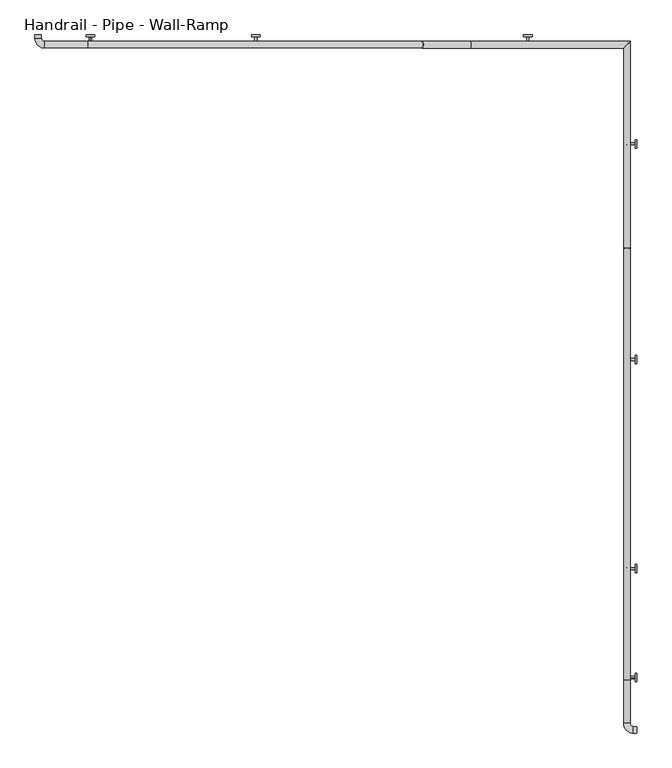
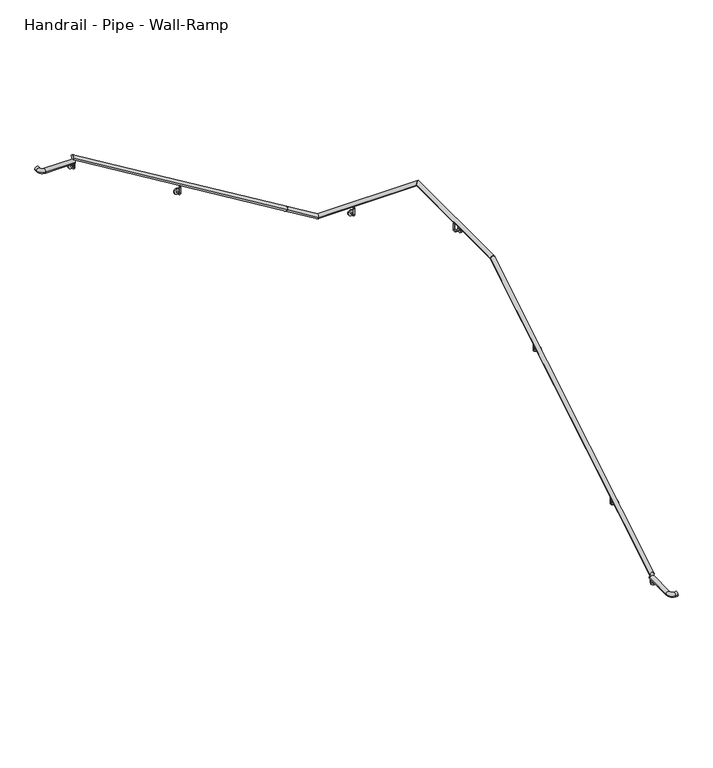
"""IFC4 building model written with IfcOpenShell, lengths in millimetres: railing geometry, Handrail - Pipe - Wall-Ramp."""

from ifc_helpers import new_model, si_unit, point, frame, frame_2d, origin, place, context, project, spatial, circle_curve, ellipse_curve, trimmed, segment, composite_curve, outline, extrude, source, transform, mapped, element, save
from ifc_brep_helpers import plane_surface, cylinder_surface, revolved_surface, advanced_brep


def handrail_pipe_wall_ramp_3ec7286e(model_context):
    return source(origin(), model_context, "Body", "SolidModel", [
        advanced_brep(
        [(-6920.3581077, -11181.433999, 1061.4577857), (-6882.2581077, -11181.433999, 1061.4577857), (-6920.3581077, -8661.5118455, 2588.6833333), (-6882.2581077, -8661.5118455, 2588.6833333)],
        [
            (0, 1, ellipse_curve(frame((-6901.3081077, -11181.433999, 1061.4577857), z_axis=(0.0, -1.0, 0.0), x_axis=(0.0, 0.0, -1.0)), 22.2755476, 19.05)),
            (1, 0, ellipse_curve(frame((-6901.3081077, -11181.433999, 1061.4577857), z_axis=(0.0, -1.0, 0.0), x_axis=(0.0, 0.0, -1.0)), 22.2755476, 19.05)),
            (2, 3, ellipse_curve(frame((-6901.3081077, -8661.5118455, 2588.6833333), z_axis=(0.0, 0.963119367356418, 0.26907449567540415), x_axis=(0.0, 0.26907449567540404, -0.9631193673564179)), 19.7794797, 19.05)),
            (3, 2, ellipse_curve(frame((-6901.3081077, -8661.5118455, 2588.6833333), z_axis=(0.0, 0.963119367356418, 0.26907449567540415), x_axis=(0.0, 0.26907449567540404, -0.9631193673564179)), 19.7794797, 19.05)),
            (0, 2),
            (3, 1),
        ],
        [
            plane_surface(frame((-6901.3081077, -11181.433999, 1083.7333333), z_axis=(0.0, -1.0, 0.0), x_axis=(0.0, 0.0, 1.0))),
            plane_surface(frame((-6901.3081077, -8666.833999, 2607.7333333), z_axis=(0.0, 0.963119367356418, 0.26907449567540415), x_axis=(1.0, 0.0, 0.0))),
            cylinder_surface(frame((-6901.3081077, -11171.5603513, 1067.4418146), z_axis=(0.0, -0.8551978315540538, -0.518301716093285), x_axis=(1.0, 0.0, 0.0)), 19.05),
        ],
        [
            (0, [[1, 2]]),
            (1, [[3, 4]]),
            (2, [[-1, 5, -4, 6]]),
            (2, [[-2, -6, -3, -5]]),
        ],
    ),
        advanced_brep(
        [(-6920.3581077, -8661.5118455, 2588.6833333), (-6882.2581077, -8661.5118455, 2588.6833333), (-6920.3581077, -7498.433999, 2588.6833333), (-6882.2581077, -7460.333999, 2588.6833333)],
        [
            (0, 1, ellipse_curve(frame((-6901.3081077, -8661.5118455, 2588.6833333), z_axis=(0.0, -0.963119367356418, -0.26907449567540415), x_axis=(0.0, -0.2690744956754042, 0.963119367356418)), 19.7794797, 19.05)),
            (1, 0, ellipse_curve(frame((-6901.3081077, -8661.5118455, 2588.6833333), z_axis=(0.0, -0.963119367356418, -0.26907449567540415), x_axis=(0.0, -0.2690744956754042, 0.963119367356418)), 19.7794797, 19.05)),
            (2, 3, ellipse_curve(frame((-6901.3081077, -7479.383999, 2588.6833333), z_axis=(-0.7071067811865462, 0.7071067811865488, 0.0), x_axis=(-0.7071067811865488, -0.7071067811865462, 0.0)), 26.9407684, 19.05)),
            (3, 2, ellipse_curve(frame((-6901.3081077, -7479.383999, 2588.6833333), z_axis=(-0.7071067811865462, 0.7071067811865488, 0.0), x_axis=(-0.7071067811865488, -0.7071067811865462, 0.0)), 26.9407684, 19.05)),
            (0, 2),
            (3, 1),
        ],
        [
            plane_surface(frame((-6901.3081077, -8666.833999, 2607.7333333), z_axis=(0.0, -0.963119367356418, -0.26907449567540415), x_axis=(1.0, 0.0, 0.0))),
            plane_surface(frame((-6901.3081077, -7479.383999, 2607.7333333), z_axis=(-0.7071067811865462, 0.7071067811865488, 0.0), x_axis=(0.7071067811865488, 0.7071067811865462, 0.0))),
            cylinder_surface(frame((-6901.3081077, -8666.833999, 2588.6833333), z_axis=(0.0, -1.0, 0.0), x_axis=(1.0, 0.0, 0.0)), 19.05),
        ],
        [
            (0, [[1, 2]]),
            (1, [[3, 4]]),
            (2, [[-1, 5, -4, 6]]),
            (2, [[-2, -6, -3, -5]]),
        ],
    ),
        advanced_brep(
        [(-6920.3581077, -7498.433999, 2588.6833333), (-6882.2581077, -7460.333999, 2588.6833333), (-7814.6802613, -7498.433999, 2588.6833333), (-7814.6802613, -7460.333999, 2588.6833333), (-8098.6317554, -7498.433999, 2760.775148), (-8098.6317554, -7460.333999, 2760.775148)],
        [
            (0, 1, ellipse_curve(frame((-6901.3081077, -7479.383999, 2588.6833333), z_axis=(0.7071067811865462, -0.7071067811865488, 0.0), x_axis=(0.7071067811865488, 0.7071067811865462, 0.0)), 26.9407684, 19.05)),
            (1, 0, ellipse_curve(frame((-6901.3081077, -7479.383999, 2588.6833333), z_axis=(0.7071067811865462, -0.7071067811865488, 0.0), x_axis=(0.7071067811865488, 0.7071067811865462, 0.0)), 26.9407684, 19.05)),
            (0, 2),
            (2, 3, ellipse_curve(frame((-7814.6802613, -7479.383999, 2588.6833333), z_axis=(0.9631193673564179, 0.0, -0.2690744956754043), x_axis=(0.2690744956754048, 0.0, 0.9631193673564179)), 19.7794797, 19.05)),
            (3, 1),
            (3, 2, ellipse_curve(frame((-7814.6802613, -7479.383999, 2588.6833333), z_axis=(0.9631193673564179, 0.0, -0.2690744956754043), x_axis=(0.2690744956754048, 0.0, 0.9631193673564179)), 19.7794797, 19.05)),
            (4, 5, circle_curve(frame((-8098.6317554, -7479.383999, 2760.775148), z_axis=(-0.8551978315540536, 0.0, 0.5183017160932853), x_axis=(0.0, 1.0, 0.0)), 19.05)),
            (5, 4, circle_curve(frame((-8098.6317554, -7479.383999, 2760.775148), z_axis=(-0.8551978315540536, 0.0, 0.5183017160932853), x_axis=(0.0, 1.0, 0.0)), 19.05)),
            (2, 4),
            (5, 3),
        ],
        [
            plane_surface(frame((-6901.3081077, -7479.383999, 2607.7333333), z_axis=(0.7071067811865462, -0.7071067811865488, 0.0), x_axis=(0.7071067811865488, 0.7071067811865462, 0.0))),
            cylinder_surface(frame((-6901.3081077, -7479.383999, 2588.6833333), z_axis=(1.0, 0.0, 0.0), x_axis=(0.0, 1.0, 0.0)), 19.05),
            plane_surface(frame((-8088.7581077, -7479.383999, 2777.0666667), z_axis=(-0.8551978315540536, 0.0, 0.5183017160932853), x_axis=(0.5183017160932853, 0.0, 0.8551978315540536))),
            cylinder_surface(frame((-7819.2317554, -7479.383999, 2591.4418146), z_axis=(0.8551978315540536, 0.0, -0.5183017160932853), x_axis=(0.0, 1.0, 0.0)), 19.05),
        ],
        [
            (0, [[1, 2]]),
            (1, [[-1, 3, 4, 5]]),
            (1, [[-2, -5, 6, -3]]),
            (2, [[7, 8]]),
            (3, [[-4, 9, -8, 10]]),
            (3, [[-6, -10, -7, -9]]),
        ],
    ),
        advanced_brep(
        [(-8098.6317554, -7498.433999, 2760.775148), (-8098.6317554, -7460.333999, 2760.775148), (-10044.5581077, -7498.433999, 3940.1244524), (-10044.5581077, -7460.333999, 3940.1244524)],
        [
            (0, 1, circle_curve(frame((-8098.6317554, -7479.383999, 2760.775148), z_axis=(0.8551978315540537, 0.0, -0.5183017160932851), x_axis=(0.0, 1.0, 0.0)), 19.05)),
            (1, 0, circle_curve(frame((-8098.6317554, -7479.383999, 2760.775148), z_axis=(0.8551978315540537, 0.0, -0.5183017160932851), x_axis=(0.0, 1.0, 0.0)), 19.05)),
            (2, 3, ellipse_curve(frame((-10044.5581077, -7479.383999, 3940.1244524), z_axis=(-1.0, 0.0, 0.0), x_axis=(0.0, 0.0, -1.0)), 22.2755476, 19.05)),
            (3, 2, ellipse_curve(frame((-10044.5581077, -7479.383999, 3940.1244524), z_axis=(-1.0, 0.0, 0.0), x_axis=(0.0, 0.0, -1.0)), 22.2755476, 19.05)),
            (0, 2),
            (3, 1),
        ],
        [
            plane_surface(frame((-8088.7581077, -7479.383999, 2777.0666667), z_axis=(0.8551978315540538, 0.0, -0.5183017160932851), x_axis=(0.5183017160932851, 0.0, 0.8551978315540538))),
            plane_surface(frame((-10044.5581077, -7479.383999, 3962.4), z_axis=(-1.0, 0.0, 0.0), x_axis=(0.0, -1.0, 0.0))),
            cylinder_surface(frame((-8098.6317554, -7479.383999, 2760.775148), z_axis=(0.8551978315540537, 0.0, -0.5183017160932851), x_axis=(0.0, 1.0, 0.0)), 19.05),
        ],
        [
            (0, [[1, 2]]),
            (1, [[3, 4]]),
            (2, [[-1, 5, -4, 6]]),
            (2, [[-2, -6, -3, -5]]),
        ],
    ),
        advanced_brep(
        [(-9060.3081077, -7479.383999, 3312.5833333), (-9073.0081077, -7479.383999, 3312.5833333), (-9060.3081077, -7479.383999, 3255.4333333), (-9073.0081077, -7479.383999, 3255.4333333), (-9073.0081077, -7460.333999, 3236.3833333), (-9060.3081077, -7460.333999, 3236.3833333), (-9060.3081077, -7431.758999, 3236.3833333), (-9073.0081077, -7431.758999, 3236.3833333)],
        [
            (0, 1, circle_curve(frame((-9066.6581077, -7479.383999, 3312.5833333), z_axis=(0.0, 0.0, 1.0), x_axis=(-1.0, 0.0, 0.0)), 6.35)),
            (1, 0, circle_curve(frame((-9066.6581077, -7479.383999, 3312.5833333), z_axis=(0.0, 0.0, 1.0), x_axis=(-1.0, 0.0, 0.0)), 6.35)),
            (0, 2),
            (2, 3, circle_curve(frame((-9066.6581077, -7479.383999, 3255.4333333), z_axis=(0.0, 0.0, 1.0), x_axis=(-1.0, 0.0, 0.0)), 6.35)),
            (3, 1),
            (3, 2, circle_curve(frame((-9066.6581077, -7479.383999, 3255.4333333), z_axis=(0.0, 0.0, 1.0), x_axis=(-1.0, 0.0, 0.0)), 6.35)),
            (4, 3, circle_curve(frame((-9073.0081077, -7460.333999, 3255.4333333), z_axis=(-1.0, 0.0, 0.0), x_axis=(0.0, -1.0, 0.0)), 19.05)),
            (2, 5, circle_curve(frame((-9060.3081077, -7460.333999, 3255.4333333), z_axis=(1.0, 0.0, 0.0), x_axis=(0.0, -1.0, 0.0)), 19.05)),
            (5, 4, circle_curve(frame((-9066.6581077, -7460.333999, 3236.3833333), z_axis=(0.0, -1.0, 0.0), x_axis=(-1.0, 0.0, 0.0)), 6.35)),
            (4, 5, circle_curve(frame((-9066.6581077, -7460.333999, 3236.3833333), z_axis=(0.0, -1.0, 0.0), x_axis=(-1.0, 0.0, 0.0)), 6.35)),
            (6, 7, circle_curve(frame((-9066.6581077, -7431.758999, 3236.3833333), z_axis=(0.0, 1.0, 0.0), x_axis=(-1.0, 0.0, 0.0)), 6.35)),
            (7, 6, circle_curve(frame((-9066.6581077, -7431.758999, 3236.3833333), z_axis=(0.0, 1.0, 0.0), x_axis=(-1.0, 0.0, 0.0)), 6.35)),
            (5, 6),
            (7, 4),
        ],
        [
            plane_surface(frame((-9073.0081077, -7479.383999, 3312.5833333), z_axis=(0.0, 0.0, 1.0), x_axis=(0.0, 1.0, 0.0))),
            cylinder_surface(frame((-9066.6581077, -7479.383999, 3312.5833333), z_axis=(0.0, 0.0, 1.0), x_axis=(-1.0, 0.0, 0.0)), 6.35),
            revolved_surface(trimmed(ellipse_curve(frame((-9066.6581077, -7479.383999, 3255.4333333), z_axis=(0.0, 0.0, 1.0), x_axis=(-1.0, 0.0, 0.0)), 6.35, 6.35), [point((-9060.3081077, -7479.383999, 3255.4333333))], [point((-9073.0081077, -7479.383999, 3255.4333333))], True, "CARTESIAN"), (-9066.6581077, -7460.333999, 3255.4333333), (1.0, 0.0, 0.0)),
            revolved_surface(trimmed(ellipse_curve(frame((-9066.6581077, -7479.383999, 3255.4333333), z_axis=(0.0, 0.0, 1.0), x_axis=(-1.0, 0.0, 0.0)), 6.35, 6.35), [point((-9073.0081077, -7479.383999, 3255.4333333))], [point((-9060.3081077, -7479.383999, 3255.4333333))], True, "CARTESIAN"), (-9066.6581077, -7460.333999, 3255.4333333), (1.0, 0.0, 0.0)),
            plane_surface(frame((-9066.6581077, -7431.758999, 3230.0333333), z_axis=(0.0, 1.0, 0.0), x_axis=(-1.0, 0.0, 0.0))),
            cylinder_surface(frame((-9066.6581077, -7460.333999, 3236.3833333), z_axis=(0.0, -1.0, 0.0), x_axis=(-1.0, 0.0, 0.0)), 6.35),
        ],
        [
            (0, [[1, 2]]),
            (1, [[-1, 3, 4, 5]]),
            (1, [[-2, -5, 6, -3]]),
            (2, [[7, -4, 8, 9]]),
            (3, [[-8, -6, -7, 10]]),
            (4, [[11, 12]]),
            (5, [[-9, 13, -12, 14]]),
            (5, [[-10, -14, -11, -13]]),
        ],
    ),
        extrude(outline(composite_curve([segment(trimmed(circle_curve(frame_2d((3236.3833333, -9066.6581077)), 25.4), [point((3236.3833333, -9092.0581077))], [point((3236.3833333, -9041.2581077))], False, "CARTESIAN"), True, "CONTINUOUS"), segment(trimmed(circle_curve(frame_2d((3236.3833333, -9066.6581077)), 25.4), [point((3236.3833333, -9041.2581077))], [point((3236.3833333, -9092.0581077))], False, "CARTESIAN"), True, "CONTINUOUS")], self_intersect=False)), frame((0.0, -7431.758999, 0.0), z_axis=(0.0, 1.0, 0.0), x_axis=(0.0, 0.0, 1.0)), (0.0, 0.0, 1.0), 9.525),
        advanced_brep(
        [(-7472.8081077, -7479.383999, 2550.5833333), (-7485.5081077, -7479.383999, 2550.5833333), (-7472.8081077, -7479.383999, 2493.4333333), (-7485.5081077, -7479.383999, 2493.4333333), (-7485.5081077, -7460.333999, 2474.3833333), (-7472.8081077, -7460.333999, 2474.3833333), (-7472.8081077, -7431.758999, 2474.3833333), (-7485.5081077, -7431.758999, 2474.3833333)],
        [
            (0, 1, circle_curve(frame((-7479.1581077, -7479.383999, 2550.5833333), z_axis=(0.0, 0.0, 1.0), x_axis=(-1.0, 0.0, 0.0)), 6.35)),
            (1, 0, circle_curve(frame((-7479.1581077, -7479.383999, 2550.5833333), z_axis=(0.0, 0.0, 1.0), x_axis=(-1.0, 0.0, 0.0)), 6.35)),
            (0, 2),
            (2, 3, circle_curve(frame((-7479.1581077, -7479.383999, 2493.4333333), z_axis=(0.0, 0.0, 1.0), x_axis=(-1.0, 0.0, 0.0)), 6.35)),
            (3, 1),
            (3, 2, circle_curve(frame((-7479.1581077, -7479.383999, 2493.4333333), z_axis=(0.0, 0.0, 1.0), x_axis=(-1.0, 0.0, 0.0)), 6.35)),
            (4, 3, circle_curve(frame((-7485.5081077, -7460.333999, 2493.4333333), z_axis=(-1.0, 0.0, 0.0), x_axis=(0.0, -1.0, 0.0)), 19.05)),
            (2, 5, circle_curve(frame((-7472.8081077, -7460.333999, 2493.4333333), z_axis=(1.0, 0.0, 0.0), x_axis=(0.0, -1.0, 0.0)), 19.05)),
            (5, 4, circle_curve(frame((-7479.1581077, -7460.333999, 2474.3833333), z_axis=(0.0, -1.0, 0.0), x_axis=(-1.0, 0.0, 0.0)), 6.35)),
            (4, 5, circle_curve(frame((-7479.1581077, -7460.333999, 2474.3833333), z_axis=(0.0, -1.0, 0.0), x_axis=(-1.0, 0.0, 0.0)), 6.35)),
            (6, 7, circle_curve(frame((-7479.1581077, -7431.758999, 2474.3833333), z_axis=(0.0, 1.0, 0.0), x_axis=(-1.0, 0.0, 0.0)), 6.35)),
            (7, 6, circle_curve(frame((-7479.1581077, -7431.758999, 2474.3833333), z_axis=(0.0, 1.0, 0.0), x_axis=(-1.0, 0.0, 0.0)), 6.35)),
            (5, 6),
            (7, 4),
        ],
        [
            plane_surface(frame((-7485.5081077, -7479.383999, 2550.5833333), z_axis=(0.0, 0.0, 1.0), x_axis=(0.0, 1.0, 0.0))),
            cylinder_surface(frame((-7479.1581077, -7479.383999, 2550.5833333), z_axis=(0.0, 0.0, 1.0), x_axis=(-1.0, 0.0, 0.0)), 6.35),
            revolved_surface(trimmed(ellipse_curve(frame((-7479.1581077, -7479.383999, 2493.4333333), z_axis=(0.0, 0.0, 1.0), x_axis=(-1.0, 0.0, 0.0)), 6.35, 6.35), [point((-7472.8081077, -7479.383999, 2493.4333333))], [point((-7485.5081077, -7479.383999, 2493.4333333))], True, "CARTESIAN"), (-7479.1581077, -7460.333999, 2493.4333333), (1.0, 0.0, 0.0)),
            revolved_surface(trimmed(ellipse_curve(frame((-7479.1581077, -7479.383999, 2493.4333333), z_axis=(0.0, 0.0, 1.0), x_axis=(-1.0, 0.0, 0.0)), 6.35, 6.35), [point((-7485.5081077, -7479.383999, 2493.4333333))], [point((-7472.8081077, -7479.383999, 2493.4333333))], True, "CARTESIAN"), (-7479.1581077, -7460.333999, 2493.4333333), (1.0, 0.0, 0.0)),
            plane_surface(frame((-7479.1581077, -7431.758999, 2468.0333333), z_axis=(0.0, 1.0, 0.0), x_axis=(-1.0, 0.0, 0.0))),
            cylinder_surface(frame((-7479.1581077, -7460.333999, 2474.3833333), z_axis=(0.0, -1.0, 0.0), x_axis=(-1.0, 0.0, 0.0)), 6.35),
        ],
        [
            (0, [[1, 2]]),
            (1, [[-1, 3, 4, 5]]),
            (1, [[-2, -5, 6, -3]]),
            (2, [[7, -4, 8, 9]]),
            (3, [[-8, -6, -7, 10]]),
            (4, [[11, 12]]),
            (5, [[-9, 13, -12, 14]]),
            (5, [[-10, -14, -11, -13]]),
        ],
    ),
        extrude(outline(composite_curve([segment(trimmed(circle_curve(frame_2d((2474.3833333, -7479.1581077)), 25.4), [point((2474.3833333, -7504.5581077))], [point((2474.3833333, -7453.7581077))], False, "CARTESIAN"), True, "CONTINUOUS"), segment(trimmed(circle_curve(frame_2d((2474.3833333, -7479.1581077)), 25.4), [point((2474.3833333, -7453.7581077))], [point((2474.3833333, -7504.5581077))], False, "CARTESIAN"), True, "CONTINUOUS")], self_intersect=False)), frame((0.0, -7431.758999, 0.0), z_axis=(0.0, 1.0, 0.0), x_axis=(0.0, 0.0, 1.0)), (0.0, 0.0, 1.0), 9.525),
        advanced_brep(
        [(-6901.3081077, -8063.583999, 2550.5833333), (-6901.3081077, -8050.883999, 2550.5833333), (-6901.3081077, -8063.583999, 2493.4333333), (-6901.3081077, -8050.883999, 2493.4333333), (-6882.2581077, -8050.883999, 2474.3833333), (-6882.2581077, -8063.583999, 2474.3833333), (-6853.6831077, -8063.583999, 2474.3833333), (-6853.6831077, -8050.883999, 2474.3833333)],
        [
            (0, 1, circle_curve(frame((-6901.3081077, -8057.233999, 2550.5833333), z_axis=(0.0, 0.0, 1.0), x_axis=(0.0, 1.0, 0.0)), 6.35)),
            (1, 0, circle_curve(frame((-6901.3081077, -8057.233999, 2550.5833333), z_axis=(0.0, 0.0, 1.0), x_axis=(0.0, 1.0, 0.0)), 6.35)),
            (0, 2),
            (2, 3, circle_curve(frame((-6901.3081077, -8057.233999, 2493.4333333), z_axis=(0.0, 0.0, 1.0), x_axis=(0.0, 1.0, 0.0)), 6.35)),
            (3, 1),
            (3, 2, circle_curve(frame((-6901.3081077, -8057.233999, 2493.4333333), z_axis=(0.0, 0.0, 1.0), x_axis=(0.0, 1.0, 0.0)), 6.35)),
            (4, 3, circle_curve(frame((-6882.2581077, -8050.883999, 2493.4333333), z_axis=(0.0, 1.0, 0.0), x_axis=(-1.0, 0.0, 0.0)), 19.05)),
            (2, 5, circle_curve(frame((-6882.2581077, -8063.583999, 2493.4333333), z_axis=(0.0, -1.0, 0.0), x_axis=(-1.0, 0.0, 0.0)), 19.05)),
            (5, 4, circle_curve(frame((-6882.2581077, -8057.233999, 2474.3833333), z_axis=(-1.0, 0.0, 0.0), x_axis=(0.0, 1.0, 0.0)), 6.35)),
            (4, 5, circle_curve(frame((-6882.2581077, -8057.233999, 2474.3833333), z_axis=(-1.0, 0.0, 0.0), x_axis=(0.0, 1.0, 0.0)), 6.35)),
            (6, 7, circle_curve(frame((-6853.6831077, -8057.233999, 2474.3833333), z_axis=(1.0, 0.0, 0.0), x_axis=(0.0, 1.0, 0.0)), 6.35)),
            (7, 6, circle_curve(frame((-6853.6831077, -8057.233999, 2474.3833333), z_axis=(1.0, 0.0, 0.0), x_axis=(0.0, 1.0, 0.0)), 6.35)),
            (5, 6),
            (7, 4),
        ],
        [
            plane_surface(frame((-6901.3081077, -8050.883999, 2550.5833333), z_axis=(0.0, 0.0, 1.0), x_axis=(1.0, 0.0, 0.0))),
            cylinder_surface(frame((-6901.3081077, -8057.233999, 2550.5833333), z_axis=(0.0, 0.0, 1.0), x_axis=(0.0, 1.0, 0.0)), 6.35),
            revolved_surface(trimmed(ellipse_curve(frame((-6901.3081077, -8057.233999, 2493.4333333), z_axis=(0.0, 0.0, 1.0), x_axis=(0.0, 1.0, 0.0)), 6.35, 6.35), [point((-6901.3081077, -8063.583999, 2493.4333333))], [point((-6901.3081077, -8050.883999, 2493.4333333))], True, "CARTESIAN"), (-6882.2581077, -8057.233999, 2493.4333333), (0.0, -1.0, 0.0)),
            revolved_surface(trimmed(ellipse_curve(frame((-6901.3081077, -8057.233999, 2493.4333333), z_axis=(0.0, 0.0, 1.0), x_axis=(0.0, 1.0, 0.0)), 6.35, 6.35), [point((-6901.3081077, -8050.883999, 2493.4333333))], [point((-6901.3081077, -8063.583999, 2493.4333333))], True, "CARTESIAN"), (-6882.2581077, -8057.233999, 2493.4333333), (0.0, -1.0, 0.0)),
            plane_surface(frame((-6853.6831077, -8057.233999, 2468.0333333), z_axis=(1.0, 0.0, 0.0), x_axis=(0.0, 1.0, 0.0))),
            cylinder_surface(frame((-6882.2581077, -8057.233999, 2474.3833333), z_axis=(-1.0, 0.0, 0.0), x_axis=(0.0, 1.0, 0.0)), 6.35),
        ],
        [
            (0, [[1, 2]]),
            (1, [[-1, 3, 4, 5]]),
            (1, [[-2, -5, 6, -3]]),
            (2, [[7, -4, 8, 9]]),
            (3, [[-8, -6, -7, 10]]),
            (4, [[11, 12]]),
            (5, [[-9, 13, -12, 14]]),
            (5, [[-10, -14, -11, -13]]),
        ],
    ),
        extrude(outline(composite_curve([segment(trimmed(circle_curve(frame_2d((-8057.233999, 2474.3833333)), 25.4), [point((-8031.833999, 2474.3833333))], [point((-8082.633999, 2474.3833333))], False, "CARTESIAN"), True, "CONTINUOUS"), segment(trimmed(circle_curve(frame_2d((-8057.233999, 2474.3833333)), 25.4), [point((-8082.633999, 2474.3833333))], [point((-8031.833999, 2474.3833333))], False, "CARTESIAN"), True, "CONTINUOUS")], self_intersect=False)), frame((-6853.6831077, 0.0, 0.0), z_axis=(1.0, 0.0, 0.0), x_axis=(0.0, 1.0, 0.0)), (0.0, 0.0, 1.0), 9.525),
        advanced_brep(
        [(-6901.3081077, -9320.883999, 2158.0378788), (-6901.3081077, -9308.183999, 2158.0378788), (-6901.3081077, -9320.883999, 2100.8878788), (-6901.3081077, -9308.183999, 2100.8878788), (-6882.2581077, -9308.183999, 2081.8378788), (-6882.2581077, -9320.883999, 2081.8378788), (-6853.6831077, -9320.883999, 2081.8378788), (-6853.6831077, -9308.183999, 2081.8378788)],
        [
            (0, 1, circle_curve(frame((-6901.3081077, -9314.533999, 2158.0378788), z_axis=(0.0, 0.0, 1.0), x_axis=(0.0, 1.0, 0.0)), 6.35)),
            (1, 0, circle_curve(frame((-6901.3081077, -9314.533999, 2158.0378788), z_axis=(0.0, 0.0, 1.0), x_axis=(0.0, 1.0, 0.0)), 6.35)),
            (0, 2),
            (2, 3, circle_curve(frame((-6901.3081077, -9314.533999, 2100.8878788), z_axis=(0.0, 0.0, 1.0), x_axis=(0.0, 1.0, 0.0)), 6.35)),
            (3, 1),
            (3, 2, circle_curve(frame((-6901.3081077, -9314.533999, 2100.8878788), z_axis=(0.0, 0.0, 1.0), x_axis=(0.0, 1.0, 0.0)), 6.35)),
            (4, 3, circle_curve(frame((-6882.2581077, -9308.183999, 2100.8878788), z_axis=(0.0, 1.0, 0.0), x_axis=(-1.0, 0.0, 0.0)), 19.05)),
            (2, 5, circle_curve(frame((-6882.2581077, -9320.883999, 2100.8878788), z_axis=(0.0, -1.0, 0.0), x_axis=(-1.0, 0.0, 0.0)), 19.05)),
            (5, 4, circle_curve(frame((-6882.2581077, -9314.533999, 2081.8378788), z_axis=(-1.0, 0.0, 0.0), x_axis=(0.0, 1.0, 0.0)), 6.35)),
            (4, 5, circle_curve(frame((-6882.2581077, -9314.533999, 2081.8378788), z_axis=(-1.0, 0.0, 0.0), x_axis=(0.0, 1.0, 0.0)), 6.35)),
            (6, 7, circle_curve(frame((-6853.6831077, -9314.533999, 2081.8378788), z_axis=(1.0, 0.0, 0.0), x_axis=(0.0, 1.0, 0.0)), 6.35)),
            (7, 6, circle_curve(frame((-6853.6831077, -9314.533999, 2081.8378788), z_axis=(1.0, 0.0, 0.0), x_axis=(0.0, 1.0, 0.0)), 6.35)),
            (5, 6),
            (7, 4),
        ],
        [
            plane_surface(frame((-6901.3081077, -9308.183999, 2158.0378788), z_axis=(0.0, 0.0, 1.0), x_axis=(1.0, 0.0, 0.0))),
            cylinder_surface(frame((-6901.3081077, -9314.533999, 2158.0378788), z_axis=(0.0, 0.0, 1.0), x_axis=(0.0, 1.0, 0.0)), 6.35),
            revolved_surface(trimmed(ellipse_curve(frame((-6901.3081077, -9314.533999, 2100.8878788), z_axis=(0.0, 0.0, 1.0), x_axis=(0.0, 1.0, 0.0)), 6.35, 6.35), [point((-6901.3081077, -9320.883999, 2100.8878788))], [point((-6901.3081077, -9308.183999, 2100.8878788))], True, "CARTESIAN"), (-6882.2581077, -9314.533999, 2100.8878788), (0.0, -1.0, 0.0)),
            revolved_surface(trimmed(ellipse_curve(frame((-6901.3081077, -9314.533999, 2100.8878788), z_axis=(0.0, 0.0, 1.0), x_axis=(0.0, 1.0, 0.0)), 6.35, 6.35), [point((-6901.3081077, -9308.183999, 2100.8878788))], [point((-6901.3081077, -9320.883999, 2100.8878788))], True, "CARTESIAN"), (-6882.2581077, -9314.533999, 2100.8878788), (0.0, -1.0, 0.0)),
            plane_surface(frame((-6853.6831077, -9314.533999, 2075.4878788), z_axis=(1.0, 0.0, 0.0), x_axis=(0.0, 1.0, 0.0))),
            cylinder_surface(frame((-6882.2581077, -9314.533999, 2081.8378788), z_axis=(-1.0, 0.0, 0.0), x_axis=(0.0, 1.0, 0.0)), 6.35),
        ],
        [
            (0, [[1, 2]]),
            (1, [[-1, 3, 4, 5]]),
            (1, [[-2, -5, 6, -3]]),
            (2, [[7, -4, 8, 9]]),
            (3, [[-8, -6, -7, 10]]),
            (4, [[11, 12]]),
            (5, [[-9, 13, -12, 14]]),
            (5, [[-10, -14, -11, -13]]),
        ],
    ),
        extrude(outline(composite_curve([segment(trimmed(circle_curve(frame_2d((-9314.533999, 2081.8378788)), 25.4), [point((-9289.133999, 2081.8378788))], [point((-9339.933999, 2081.8378788))], False, "CARTESIAN"), True, "CONTINUOUS"), segment(trimmed(circle_curve(frame_2d((-9314.533999, 2081.8378788)), 25.4), [point((-9339.933999, 2081.8378788))], [point((-9289.133999, 2081.8378788))], False, "CARTESIAN"), True, "CONTINUOUS")], self_intersect=False)), frame((-6853.6831077, 0.0, 0.0), z_axis=(1.0, 0.0, 0.0), x_axis=(0.0, 1.0, 0.0)), (0.0, 0.0, 1.0), 9.525),
        advanced_brep(
        [(-6901.3081077, -10540.083999, 1419.1287879), (-6901.3081077, -10527.383999, 1419.1287879), (-6901.3081077, -10540.083999, 1361.9787879), (-6901.3081077, -10527.383999, 1361.9787879), (-6882.2581077, -10527.383999, 1342.9287879), (-6882.2581077, -10540.083999, 1342.9287879), (-6853.6831077, -10540.083999, 1342.9287879), (-6853.6831077, -10527.383999, 1342.9287879)],
        [
            (0, 1, circle_curve(frame((-6901.3081077, -10533.733999, 1419.1287879), z_axis=(0.0, 0.0, 1.0), x_axis=(0.0, 1.0, 0.0)), 6.35)),
            (1, 0, circle_curve(frame((-6901.3081077, -10533.733999, 1419.1287879), z_axis=(0.0, 0.0, 1.0), x_axis=(0.0, 1.0, 0.0)), 6.35)),
            (0, 2),
            (2, 3, circle_curve(frame((-6901.3081077, -10533.733999, 1361.9787879), z_axis=(0.0, 0.0, 1.0), x_axis=(0.0, 1.0, 0.0)), 6.35)),
            (3, 1),
            (3, 2, circle_curve(frame((-6901.3081077, -10533.733999, 1361.9787879), z_axis=(0.0, 0.0, 1.0), x_axis=(0.0, 1.0, 0.0)), 6.35)),
            (4, 3, circle_curve(frame((-6882.2581077, -10527.383999, 1361.9787879), z_axis=(0.0, 1.0, 0.0), x_axis=(-1.0, 0.0, 0.0)), 19.05)),
            (2, 5, circle_curve(frame((-6882.2581077, -10540.083999, 1361.9787879), z_axis=(0.0, -1.0, 0.0), x_axis=(-1.0, 0.0, 0.0)), 19.05)),
            (5, 4, circle_curve(frame((-6882.2581077, -10533.733999, 1342.9287879), z_axis=(-1.0, 0.0, 0.0), x_axis=(0.0, 1.0, 0.0)), 6.35)),
            (4, 5, circle_curve(frame((-6882.2581077, -10533.733999, 1342.9287879), z_axis=(-1.0, 0.0, 0.0), x_axis=(0.0, 1.0, 0.0)), 6.35)),
            (6, 7, circle_curve(frame((-6853.6831077, -10533.733999, 1342.9287879), z_axis=(1.0, 0.0, 0.0), x_axis=(0.0, 1.0, 0.0)), 6.35)),
            (7, 6, circle_curve(frame((-6853.6831077, -10533.733999, 1342.9287879), z_axis=(1.0, 0.0, 0.0), x_axis=(0.0, 1.0, 0.0)), 6.35)),
            (5, 6),
            (7, 4),
        ],
        [
            plane_surface(frame((-6901.3081077, -10527.383999, 1419.1287879), z_axis=(0.0, 0.0, 1.0), x_axis=(1.0, 0.0, 0.0))),
            cylinder_surface(frame((-6901.3081077, -10533.733999, 1419.1287879), z_axis=(0.0, 0.0, 1.0), x_axis=(0.0, 1.0, 0.0)), 6.35),
            revolved_surface(trimmed(ellipse_curve(frame((-6901.3081077, -10533.733999, 1361.9787879), z_axis=(0.0, 0.0, 1.0), x_axis=(0.0, 1.0, 0.0)), 6.35, 6.35), [point((-6901.3081077, -10540.083999, 1361.9787879))], [point((-6901.3081077, -10527.383999, 1361.9787879))], True, "CARTESIAN"), (-6882.2581077, -10533.733999, 1361.9787879), (0.0, -1.0, 0.0)),
            revolved_surface(trimmed(ellipse_curve(frame((-6901.3081077, -10533.733999, 1361.9787879), z_axis=(0.0, 0.0, 1.0), x_axis=(0.0, 1.0, 0.0)), 6.35, 6.35), [point((-6901.3081077, -10527.383999, 1361.9787879))], [point((-6901.3081077, -10540.083999, 1361.9787879))], True, "CARTESIAN"), (-6882.2581077, -10533.733999, 1361.9787879), (0.0, -1.0, 0.0)),
            plane_surface(frame((-6853.6831077, -10533.733999, 1336.5787879), z_axis=(1.0, 0.0, 0.0), x_axis=(0.0, 1.0, 0.0))),
            cylinder_surface(frame((-6882.2581077, -10533.733999, 1342.9287879), z_axis=(-1.0, 0.0, 0.0), x_axis=(0.0, 1.0, 0.0)), 6.35),
        ],
        [
            (0, [[1, 2]]),
            (1, [[-1, 3, 4, 5]]),
            (1, [[-2, -5, 6, -3]]),
            (2, [[7, -4, 8, 9]]),
            (3, [[-8, -6, -7, 10]]),
            (4, [[11, 12]]),
            (5, [[-9, 13, -12, 14]]),
            (5, [[-10, -14, -11, -13]]),
        ],
    ),
        extrude(outline(composite_curve([segment(trimmed(circle_curve(frame_2d((-10533.733999, 1342.9287879)), 25.4), [point((-10508.333999, 1342.9287879))], [point((-10559.133999, 1342.9287879))], False, "CARTESIAN"), True, "CONTINUOUS"), segment(trimmed(circle_curve(frame_2d((-10533.733999, 1342.9287879)), 25.4), [point((-10559.133999, 1342.9287879))], [point((-10508.333999, 1342.9287879))], False, "CARTESIAN"), True, "CONTINUOUS")], self_intersect=False)), frame((-6853.6831077, 0.0, 0.0), z_axis=(1.0, 0.0, 0.0), x_axis=(0.0, 1.0, 0.0)), (0.0, 0.0, 1.0), 9.525),
        advanced_brep(
        [(-10031.8581077, -7460.333999, 3897.5530303), (-10031.8581077, -7498.433999, 3897.5530303), (-10298.5581077, -7460.333999, 3897.5530303), (-10298.5581077, -7498.433999, 3897.5530303), (-10317.6081077, -7422.233999, 3897.5530303), (-10355.7081077, -7422.233999, 3897.5530303), (-10355.7081077, -7441.283999, 3897.5530303), (-10317.6081077, -7441.283999, 3897.5530303)],
        [
            (0, 1, circle_curve(frame((-10031.8581077, -7479.383999, 3897.5530303), z_axis=(1.0, 0.0, 0.0), x_axis=(0.0, -1.0, 0.0)), 19.05)),
            (1, 0, circle_curve(frame((-10031.8581077, -7479.383999, 3897.5530303), z_axis=(1.0, 0.0, 0.0), x_axis=(0.0, -1.0, 0.0)), 19.05)),
            (0, 2),
            (2, 3, circle_curve(frame((-10298.5581077, -7479.383999, 3897.5530303), z_axis=(1.0, 0.0, 0.0), x_axis=(0.0, -1.0, 0.0)), 19.05)),
            (3, 1),
            (3, 2, circle_curve(frame((-10298.5581077, -7479.383999, 3897.5530303), z_axis=(1.0, 0.0, 0.0), x_axis=(0.0, -1.0, 0.0)), 19.05)),
            (4, 5, circle_curve(frame((-10336.6581077, -7422.233999, 3897.5530303), z_axis=(0.0, 1.0, 0.0), x_axis=(-1.0, 0.0, 0.0)), 19.05)),
            (5, 4, circle_curve(frame((-10336.6581077, -7422.233999, 3897.5530303), z_axis=(0.0, 1.0, 0.0), x_axis=(-1.0, 0.0, 0.0)), 19.05)),
            (6, 7, circle_curve(frame((-10336.6581077, -7441.283999, 3897.5530303), z_axis=(0.0, 1.0, 0.0), x_axis=(-1.0, 0.0, 0.0)), 19.05)),
            (7, 4),
            (5, 6),
            (7, 6, circle_curve(frame((-10336.6581077, -7441.283999, 3897.5530303), z_axis=(0.0, 1.0, 0.0), x_axis=(-1.0, 0.0, 0.0)), 19.05)),
            (6, 3, circle_curve(frame((-10298.5581077, -7441.283999, 3897.5530303), z_axis=(0.0, 0.0, 1.0), x_axis=(0.0, -1.0, 0.0)), 57.15)),
            (2, 7, circle_curve(frame((-10298.5581077, -7441.283999, 3897.5530303), z_axis=(0.0, 0.0, -1.0), x_axis=(0.0, -1.0, 0.0)), 19.05)),
        ],
        [
            plane_surface(frame((-10031.8581077, -7479.383999, 3897.5530303), z_axis=(1.0, 0.0, 0.0), x_axis=(0.0, 0.0, 1.0))),
            cylinder_surface(frame((-10031.8581077, -7479.383999, 3897.5530303), z_axis=(1.0, 0.0, 0.0), x_axis=(0.0, -1.0, 0.0)), 19.05),
            plane_surface(frame((-10336.6581077, -7422.233999, 3897.5530303), z_axis=(0.0, 1.0, 0.0), x_axis=(0.0, 0.0, 1.0))),
            cylinder_surface(frame((-10336.6581077, -7441.283999, 3897.5530303), z_axis=(0.0, -1.0, 0.0), x_axis=(-1.0, 0.0, 0.0)), 19.05),
            revolved_surface(trimmed(ellipse_curve(frame((-10298.5581077, -7479.383999, 3897.5530303), z_axis=(1.0, 0.0, 0.0), x_axis=(0.0, -1.0, 0.0)), 19.05, 19.05), [point((-10298.5581077, -7460.333999, 3897.5530303))], [point((-10298.5581077, -7498.433999, 3897.5530303))], True, "CARTESIAN"), (-10298.5581077, -7441.283999, 3897.5530303), (0.0, 0.0, -1.0)),
            revolved_surface(trimmed(ellipse_curve(frame((-10298.5581077, -7479.383999, 3897.5530303), z_axis=(1.0, 0.0, 0.0), x_axis=(0.0, -1.0, 0.0)), 19.05, 19.05), [point((-10298.5581077, -7498.433999, 3897.5530303))], [point((-10298.5581077, -7460.333999, 3897.5530303))], True, "CARTESIAN"), (-10298.5581077, -7441.283999, 3897.5530303), (0.0, 0.0, -1.0)),
        ],
        [
            (0, [[1, 2]]),
            (1, [[-1, 3, 4, 5]]),
            (1, [[-2, -5, 6, -3]]),
            (2, [[7, 8]]),
            (3, [[9, 10, -8, 11]]),
            (3, [[12, -11, -7, -10]]),
            (4, [[13, -4, 14, -9]]),
            (5, [[-14, -6, -13, -12]]),
        ],
    ),
        advanced_brep(
        [(-10031.8581077, -7431.758999, 3815.0030303), (-10031.8581077, -7431.758999, 3827.7030303), (-10031.8581077, -7460.333999, 3815.0030303), (-10031.8581077, -7460.333999, 3827.7030303), (-10031.8581077, -7485.733999, 3897.5530303), (-10031.8581077, -7473.033999, 3897.5530303), (-10031.8581077, -7473.033999, 3840.4030303), (-10031.8581077, -7485.733999, 3840.4030303)],
        [
            (0, 1, circle_curve(frame((-10031.8581077, -7431.758999, 3821.3530303), z_axis=(0.0, 1.0, 0.0), x_axis=(0.0, 0.0, 1.0)), 6.35)),
            (1, 0, circle_curve(frame((-10031.8581077, -7431.758999, 3821.3530303), z_axis=(0.0, 1.0, 0.0), x_axis=(0.0, 0.0, 1.0)), 6.35)),
            (0, 2),
            (2, 3, circle_curve(frame((-10031.8581077, -7460.333999, 3821.3530303), z_axis=(0.0, 1.0, 0.0), x_axis=(0.0, 0.0, 1.0)), 6.35)),
            (3, 1),
            (3, 2, circle_curve(frame((-10031.8581077, -7460.333999, 3821.3530303), z_axis=(0.0, 1.0, 0.0), x_axis=(0.0, 0.0, 1.0)), 6.35)),
            (4, 5, circle_curve(frame((-10031.8581077, -7479.383999, 3897.5530303), z_axis=(0.0, 0.0, 1.0), x_axis=(0.0, 1.0, 0.0)), 6.35)),
            (5, 4, circle_curve(frame((-10031.8581077, -7479.383999, 3897.5530303), z_axis=(0.0, 0.0, 1.0), x_axis=(0.0, 1.0, 0.0)), 6.35)),
            (6, 7, circle_curve(frame((-10031.8581077, -7479.383999, 3840.4030303), z_axis=(0.0, 0.0, 1.0), x_axis=(0.0, 1.0, 0.0)), 6.35)),
            (7, 4),
            (5, 6),
            (7, 6, circle_curve(frame((-10031.8581077, -7479.383999, 3840.4030303), z_axis=(0.0, 0.0, 1.0), x_axis=(0.0, 1.0, 0.0)), 6.35)),
            (6, 3, circle_curve(frame((-10031.8581077, -7460.333999, 3840.4030303), z_axis=(1.0, 0.0, 0.0), x_axis=(0.0, 0.0, -1.0)), 12.7)),
            (2, 7, circle_curve(frame((-10031.8581077, -7460.333999, 3840.4030303), z_axis=(-1.0, 0.0, 0.0), x_axis=(0.0, 0.0, -1.0)), 25.4)),
        ],
        [
            plane_surface(frame((-10031.8581077, -7431.758999, 3821.3530303), z_axis=(0.0, 1.0, 0.0), x_axis=(-1.0, 0.0, 0.0))),
            cylinder_surface(frame((-10031.8581077, -7431.758999, 3821.3530303), z_axis=(0.0, 1.0, 0.0), x_axis=(0.0, 0.0, 1.0)), 6.35),
            plane_surface(frame((-10031.8581077, -7479.383999, 3897.5530303), z_axis=(0.0, 0.0, 1.0), x_axis=(-1.0, 0.0, 0.0))),
            cylinder_surface(frame((-10031.8581077, -7479.383999, 3840.4030303), z_axis=(0.0, 0.0, -1.0), x_axis=(0.0, 1.0, 0.0)), 6.35),
            revolved_surface(trimmed(ellipse_curve(frame((-10031.8581077, -7460.333999, 3821.3530303), z_axis=(0.0, 1.0, 0.0), x_axis=(0.0, 0.0, 1.0)), 6.35, 6.35), [point((-10031.8581077, -7460.333999, 3815.0030303))], [point((-10031.8581077, -7460.333999, 3827.7030303))], True, "CARTESIAN"), (-10031.8581077, -7460.333999, 3840.4030303), (-1.0, 0.0, 0.0)),
            revolved_surface(trimmed(ellipse_curve(frame((-10031.8581077, -7460.333999, 3821.3530303), z_axis=(0.0, 1.0, 0.0), x_axis=(0.0, 0.0, 1.0)), 6.35, 6.35), [point((-10031.8581077, -7460.333999, 3827.7030303))], [point((-10031.8581077, -7460.333999, 3815.0030303))], True, "CARTESIAN"), (-10031.8581077, -7460.333999, 3840.4030303), (-1.0, 0.0, 0.0)),
        ],
        [
            (0, [[1, 2]]),
            (1, [[-1, 3, 4, 5]]),
            (1, [[-2, -5, 6, -3]]),
            (2, [[7, 8]]),
            (3, [[9, 10, -8, 11]]),
            (3, [[12, -11, -7, -10]]),
            (4, [[13, -4, 14, -9]]),
            (5, [[-14, -6, -13, -12]]),
        ],
    ),
        extrude(outline(composite_curve([segment(trimmed(circle_curve(frame_2d((3821.3530303, -10031.8581077)), 25.4), [point((3821.3530303, -10057.2581077))], [point((3821.3530303, -10006.4581077))], False, "CARTESIAN"), True, "CONTINUOUS"), segment(trimmed(circle_curve(frame_2d((3821.3530303, -10031.8581077)), 25.4), [point((3821.3530303, -10006.4581077))], [point((3821.3530303, -10057.2581077))], False, "CARTESIAN"), True, "CONTINUOUS")], self_intersect=False)), frame((0.0, -7431.758999, 0.0), z_axis=(0.0, 1.0, 0.0), x_axis=(0.0, 0.0, 1.0)), (0.0, 0.0, 1.0), 9.525),
        advanced_brep(
        [(-6844.1581077, -11454.483999, 1034.280303), (-6844.1581077, -11492.583999, 1034.280303), (-6863.2081077, -11454.483999, 1034.280303), (-6863.2081077, -11492.583999, 1034.280303), (-6920.3581077, -11435.433999, 1034.280303), (-6882.2581077, -11435.433999, 1034.280303), (-6882.2581077, -11168.733999, 1034.280303), (-6920.3581077, -11168.733999, 1034.280303)],
        [
            (0, 1, circle_curve(frame((-6844.1581077, -11473.533999, 1034.280303), z_axis=(1.0, 0.0, 0.0), x_axis=(0.0, -1.0, 0.0)), 19.05)),
            (1, 0, circle_curve(frame((-6844.1581077, -11473.533999, 1034.280303), z_axis=(1.0, 0.0, 0.0), x_axis=(0.0, -1.0, 0.0)), 19.05)),
            (0, 2),
            (2, 3, circle_curve(frame((-6863.2081077, -11473.533999, 1034.280303), z_axis=(1.0, 0.0, 0.0), x_axis=(0.0, -1.0, 0.0)), 19.05)),
            (3, 1),
            (3, 2, circle_curve(frame((-6863.2081077, -11473.533999, 1034.280303), z_axis=(1.0, 0.0, 0.0), x_axis=(0.0, -1.0, 0.0)), 19.05)),
            (4, 3, circle_curve(frame((-6863.2081077, -11435.433999, 1034.280303), z_axis=(0.0, 0.0, 1.0), x_axis=(0.0, -1.0, 0.0)), 57.15)),
            (2, 5, circle_curve(frame((-6863.2081077, -11435.433999, 1034.280303), z_axis=(0.0, 0.0, -1.0), x_axis=(0.0, -1.0, 0.0)), 19.05)),
            (5, 4, circle_curve(frame((-6901.3081077, -11435.433999, 1034.280303), z_axis=(0.0, -1.0, 0.0), x_axis=(-1.0, 0.0, 0.0)), 19.05)),
            (4, 5, circle_curve(frame((-6901.3081077, -11435.433999, 1034.280303), z_axis=(0.0, -1.0, 0.0), x_axis=(-1.0, 0.0, 0.0)), 19.05)),
            (6, 7, circle_curve(frame((-6901.3081077, -11168.733999, 1034.280303), z_axis=(0.0, 1.0, 0.0), x_axis=(-1.0, 0.0, 0.0)), 19.05)),
            (7, 6, circle_curve(frame((-6901.3081077, -11168.733999, 1034.280303), z_axis=(0.0, 1.0, 0.0), x_axis=(-1.0, 0.0, 0.0)), 19.05)),
            (5, 6),
            (7, 4),
        ],
        [
            plane_surface(frame((-6844.1581077, -11473.533999, 1034.280303), z_axis=(1.0, 0.0, 0.0), x_axis=(0.0, 0.0, 1.0))),
            cylinder_surface(frame((-6844.1581077, -11473.533999, 1034.280303), z_axis=(1.0, 0.0, 0.0), x_axis=(0.0, -1.0, 0.0)), 19.05),
            revolved_surface(trimmed(ellipse_curve(frame((-6863.2081077, -11473.533999, 1034.280303), z_axis=(1.0, 0.0, 0.0), x_axis=(0.0, -1.0, 0.0)), 19.05, 19.05), [point((-6863.2081077, -11454.483999, 1034.280303))], [point((-6863.2081077, -11492.583999, 1034.280303))], True, "CARTESIAN"), (-6863.2081077, -11435.433999, 1034.280303), (0.0, 0.0, -1.0)),
            revolved_surface(trimmed(ellipse_curve(frame((-6863.2081077, -11473.533999, 1034.280303), z_axis=(1.0, 0.0, 0.0), x_axis=(0.0, -1.0, 0.0)), 19.05, 19.05), [point((-6863.2081077, -11492.583999, 1034.280303))], [point((-6863.2081077, -11454.483999, 1034.280303))], True, "CARTESIAN"), (-6863.2081077, -11435.433999, 1034.280303), (0.0, 0.0, -1.0)),
            plane_surface(frame((-6901.3081077, -11168.733999, 1034.280303), z_axis=(0.0, 1.0, 0.0), x_axis=(0.0, 0.0, 1.0))),
            cylinder_surface(frame((-6901.3081077, -11435.433999, 1034.280303), z_axis=(0.0, -1.0, 0.0), x_axis=(-1.0, 0.0, 0.0)), 19.05),
        ],
        [
            (0, [[1, 2]]),
            (1, [[-1, 3, 4, 5]]),
            (1, [[-2, -5, 6, -3]]),
            (2, [[7, -4, 8, 9]]),
            (3, [[-8, -6, -7, 10]]),
            (4, [[11, 12]]),
            (5, [[-9, 13, -12, 14]]),
            (5, [[-10, -14, -11, -13]]),
        ],
    ),
        advanced_brep(
        [(-6853.6831077, -11168.733999, 951.730303), (-6853.6831077, -11168.733999, 964.430303), (-6882.2581077, -11168.733999, 951.730303), (-6882.2581077, -11168.733999, 964.430303), (-6894.9581077, -11168.733999, 977.130303), (-6907.6581077, -11168.733999, 977.130303), (-6907.6581077, -11168.733999, 1034.280303), (-6894.9581077, -11168.733999, 1034.280303)],
        [
            (0, 1, circle_curve(frame((-6853.6831077, -11168.733999, 958.080303), z_axis=(1.0, 0.0, 0.0), x_axis=(0.0, 0.0, 1.0)), 6.35)),
            (1, 0, circle_curve(frame((-6853.6831077, -11168.733999, 958.080303), z_axis=(1.0, 0.0, 0.0), x_axis=(0.0, 0.0, 1.0)), 6.35)),
            (0, 2),
            (2, 3, circle_curve(frame((-6882.2581077, -11168.733999, 958.080303), z_axis=(1.0, 0.0, 0.0), x_axis=(0.0, 0.0, 1.0)), 6.35)),
            (3, 1),
            (3, 2, circle_curve(frame((-6882.2581077, -11168.733999, 958.080303), z_axis=(1.0, 0.0, 0.0), x_axis=(0.0, 0.0, 1.0)), 6.35)),
            (4, 3, circle_curve(frame((-6882.2581077, -11168.733999, 977.130303), z_axis=(0.0, -1.0, 0.0), x_axis=(0.0, 0.0, -1.0)), 12.7)),
            (2, 5, circle_curve(frame((-6882.2581077, -11168.733999, 977.130303), z_axis=(0.0, 1.0, 0.0), x_axis=(0.0, 0.0, -1.0)), 25.4)),
            (5, 4, circle_curve(frame((-6901.3081077, -11168.733999, 977.130303), z_axis=(0.0, 0.0, -1.0), x_axis=(1.0, 0.0, 0.0)), 6.35)),
            (4, 5, circle_curve(frame((-6901.3081077, -11168.733999, 977.130303), z_axis=(0.0, 0.0, -1.0), x_axis=(1.0, 0.0, 0.0)), 6.35)),
            (6, 7, circle_curve(frame((-6901.3081077, -11168.733999, 1034.280303), z_axis=(0.0, 0.0, 1.0), x_axis=(1.0, 0.0, 0.0)), 6.35)),
            (7, 6, circle_curve(frame((-6901.3081077, -11168.733999, 1034.280303), z_axis=(0.0, 0.0, 1.0), x_axis=(1.0, 0.0, 0.0)), 6.35)),
            (5, 6),
            (7, 4),
        ],
        [
            plane_surface(frame((-6853.6831077, -11168.733999, 958.080303), z_axis=(1.0, 0.0, 0.0), x_axis=(0.0, 1.0, 0.0))),
            cylinder_surface(frame((-6853.6831077, -11168.733999, 958.080303), z_axis=(1.0, 0.0, 0.0), x_axis=(0.0, 0.0, 1.0)), 6.35),
            revolved_surface(trimmed(ellipse_curve(frame((-6882.2581077, -11168.733999, 958.080303), z_axis=(1.0, 0.0, 0.0), x_axis=(0.0, 0.0, 1.0)), 6.35, 6.35), [point((-6882.2581077, -11168.733999, 951.730303))], [point((-6882.2581077, -11168.733999, 964.430303))], True, "CARTESIAN"), (-6882.2581077, -11168.733999, 977.130303), (0.0, 1.0, 0.0)),
            revolved_surface(trimmed(ellipse_curve(frame((-6882.2581077, -11168.733999, 958.080303), z_axis=(1.0, 0.0, 0.0), x_axis=(0.0, 0.0, 1.0)), 6.35, 6.35), [point((-6882.2581077, -11168.733999, 964.430303))], [point((-6882.2581077, -11168.733999, 951.730303))], True, "CARTESIAN"), (-6882.2581077, -11168.733999, 977.130303), (0.0, 1.0, 0.0)),
            plane_surface(frame((-6901.3081077, -11168.733999, 1034.280303), z_axis=(0.0, 0.0, 1.0), x_axis=(0.0, 1.0, 0.0))),
            cylinder_surface(frame((-6901.3081077, -11168.733999, 977.130303), z_axis=(0.0, 0.0, -1.0), x_axis=(1.0, 0.0, 0.0)), 6.35),
        ],
        [
            (0, [[1, 2]]),
            (1, [[-1, 3, 4, 5]]),
            (1, [[-2, -5, 6, -3]]),
            (2, [[7, -4, 8, 9]]),
            (3, [[-8, -6, -7, 10]]),
            (4, [[11, 12]]),
            (5, [[-9, 13, -12, 14]]),
            (5, [[-10, -14, -11, -13]]),
        ],
    ),
        extrude(outline(composite_curve([segment(trimmed(circle_curve(frame_2d((-11168.733999, 958.080303)), 25.4), [point((-11143.333999, 958.080303))], [point((-11194.133999, 958.080303))], False, "CARTESIAN"), True, "CONTINUOUS"), segment(trimmed(circle_curve(frame_2d((-11168.733999, 958.080303)), 25.4), [point((-11194.133999, 958.080303))], [point((-11143.333999, 958.080303))], False, "CARTESIAN"), True, "CONTINUOUS")], self_intersect=False)), frame((-6853.6831077, 0.0, 0.0), z_axis=(1.0, 0.0, 0.0), x_axis=(0.0, 1.0, 0.0)), (0.0, 0.0, 1.0), 9.525),
    ])


if __name__ == "__main__":
    model = new_model("IFC4")
    model_context = context("Model", 3, world=origin())
    ifc_project = project(units=[si_unit("LENGTHUNIT", "METRE", prefix="MILLI")], contexts=[model_context])
    site = spatial("IfcSite", under=ifc_project)
    building = spatial("IfcBuilding", under=site)
    placement = place(None, origin())
    handrail_pipe_wall_ramp_shape = handrail_pipe_wall_ramp_3ec7286e(model_context)
    element("IfcRailing", 1, ObjectType="Handrail - Pipe - Wall-Ramp", at=placement, inside=building, context=model_context, shape_type="MappedRepresentation", body=[
        mapped(handrail_pipe_wall_ramp_shape, transform((0.0, 0.0, 0.0), x_axis=(1.0, 0.0, 0.0), y_axis=(0.0, 1.0, 0.0), z_axis=(0.0, 0.0, 1.0))),
    ])
    save(model, "model.ifc")
